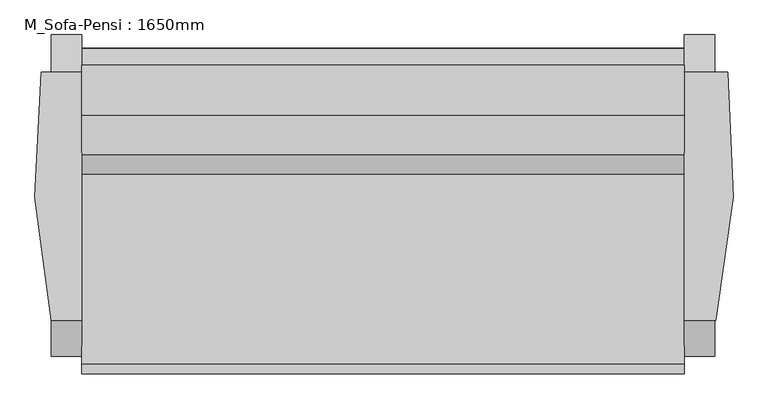
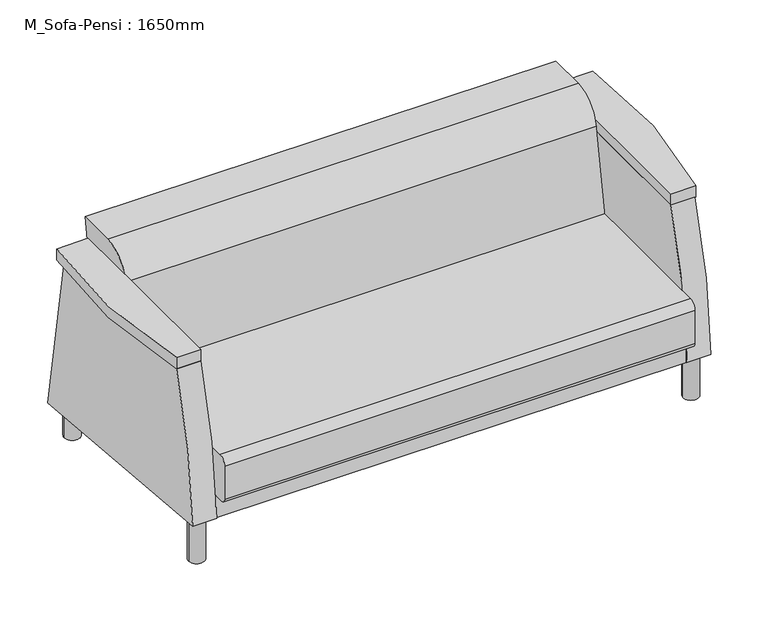
"""IFC4 building model written with IfcOpenShell, lengths in millimetres: furniture geometry, M_Sofa-Pensi : 1650mm."""

from ifc_helpers import new_model, si_unit, point, frame, frame_2d, origin, origin_with_axes, place, context, project, spatial, polyline, circle_curve, trimmed, segment, composite_curve, outline, extrude, source, transform, mapped, element, save
from ifc_brep_helpers import plane_surface, cylinder_surface, advanced_brep


def m_sofa_pensi_1650mm_31461fb8(model_context):
    return source(origin(), model_context, "Body", "SolidModel", [
        advanced_brep(
        [(1103.60625, 701.7619204, 79.3588346), (1103.60625, 608.6917937, 626.0203985), (1103.60625, -9.3943348, 626.0203985), (1103.60625, -97.7900405, 149.3105671), (1027.40625, -9.3943348, 626.0203985), (1027.40625, 608.6917937, 626.0203985), (1027.40625, 701.7619204, 79.3588346), (1027.40625, -83.3930704, 148.0509954), (1027.40625, 668.3047863, 148.0509954), (1027.40625, 668.3047863, 224.2509954), (1027.40625, -93.6952137, 224.2509954), (1027.40625, -93.6952137, 148.9523161), (1027.40625, -97.7900405, 149.3105671), (1027.40625, -93.6952137, 148.0509954), (-470.19375, -83.3930704, 148.0509954), (-470.19375, -93.6952137, 148.0509954), (-470.19375, -93.6952137, 148.9523161), (-470.19375, 668.3047863, 224.2509954), (-470.19375, -93.6952137, 224.2509954), (-470.19375, 668.3047863, 148.0509954), (-470.19375, 701.7619204, 79.3588346), (-470.19375, 608.6917937, 626.0203985), (-470.19375, -9.3943348, 626.0203985), (-470.19375, -97.7900405, 149.3105671), (-546.39375, -9.3943348, 626.0203985), (-546.39375, 608.6917937, 626.0203985), (-546.39375, 701.7619204, 79.3588346), (-546.39375, -97.7900405, 149.3105671)],
        [
            (0, 1),
            (1, 2),
            (2, 3, circle_curve(frame((1103.60625, 1499.9783711, 99.5888442), z_axis=(1.0, 0.0, 0.0), x_axis=(0.0, 1.0, 0.0)), 1598.5418814)),
            (3, 0),
            (4, 5),
            (5, 6),
            (6, 7),
            (7, 8),
            (8, 9),
            (9, 10),
            (10, 4, circle_curve(frame((1027.40625, 1499.9783711, 99.5888442), z_axis=(-1.0, 0.0, 0.0), x_axis=(0.0, 1.0, 0.0)), 1598.5418814)),
            (11, 12),
            (12, 10, circle_curve(frame((1027.40625, 1499.9783711, 99.5888442), z_axis=(-1.0, 0.0, 0.0), x_axis=(0.0, 1.0, 0.0)), 1598.5418814)),
            (10, 11),
            (0, 6),
            (5, 1),
            (4, 2),
            (12, 3),
            (11, 7),
            (11, 13),
            (13, 7),
            (14, 15),
            (15, 16),
            (16, 14),
            (9, 17),
            (17, 18),
            (18, 10),
            (18, 16),
            (15, 13),
            (14, 19),
            (19, 8),
            (19, 17),
            (20, 21),
            (21, 22),
            (22, 18, circle_curve(frame((-470.19375, 1499.9783711, 99.5888442), z_axis=(1.0, 0.0, 0.0), x_axis=(0.0, 1.0, 0.0)), 1598.5418814)),
            (14, 20),
            (18, 23, circle_curve(frame((-470.19375, 1499.9783711, 99.5888442), z_axis=(1.0, 0.0, 0.0), x_axis=(0.0, 1.0, 0.0)), 1598.5418814)),
            (23, 16),
            (24, 25),
            (25, 26),
            (26, 27),
            (27, 24, circle_curve(frame((-546.39375, 1499.9783711, 99.5888442), z_axis=(-1.0, 0.0, 0.0), x_axis=(0.0, 1.0, 0.0)), 1598.5418814)),
            (27, 23),
            (22, 24),
            (26, 20),
            (25, 21),
        ],
        [
            plane_surface(frame((1103.60625, 608.6917937, 626.0203985), z_axis=(1.0000000000000002, 0.0, 0.0), x_axis=(0.0, -0.16783676484789783, 0.985814800236531))),
            plane_surface(frame((1027.40625, 608.6917937, 626.0203985), z_axis=(-1.0000000000000002, 0.0, 0.0), x_axis=(0.0, 0.16783676484789783, -0.985814800236531))),
            plane_surface(frame((1103.60625, 701.7619204, 79.3588346), z_axis=(0.0, 0.985814800236531, 0.16783676484789783), x_axis=(-1.0, 0.0, 0.0))),
            plane_surface(frame((1103.60625, 608.6917937, 626.0203985), z_axis=(0.0, 0.0, 1.0), x_axis=(-1.0, 0.0, 0.0))),
            cylinder_surface(frame((1027.40625, 1499.9783711, 99.5888442), z_axis=(1.0, 0.0, 0.0), x_axis=(0.0, 1.0, 0.0)), 1598.5418814),
            plane_surface(frame((1103.60625, -97.7900405, 149.3105671), z_axis=(0.0, -0.08715574274767213, -0.9961946980917444), x_axis=(-1.0, 0.0, 0.0))),
            plane_surface(frame((1027.40625, -93.6952137, 224.2509954), z_axis=(1.0, 0.0, 0.0), x_axis=(0.0, -1.0, 0.0))),
            plane_surface(frame((-470.19375, -93.6952137, 224.2509954), z_axis=(-1.0, 0.0, 0.0), x_axis=(0.0, 1.0, 0.0))),
            plane_surface(frame((1027.40625, 668.3047863, 224.2509954), z_axis=(0.0, 0.0, 1.0), x_axis=(-1.0, 0.0, 0.0))),
            plane_surface(frame((1027.40625, -93.6952137, 224.2509954), z_axis=(0.0, -1.0, 0.0), x_axis=(-1.0, 0.0, 0.0))),
            plane_surface(frame((1027.40625, -93.6952137, 148.0509954), z_axis=(0.0, 0.0, -1.0), x_axis=(-1.0, 0.0, 0.0))),
            plane_surface(frame((1027.40625, 668.3047863, 148.0509954), z_axis=(0.0, 1.0, 0.0), x_axis=(-1.0, 0.0, 0.0))),
            plane_surface(frame((-470.19375, 3098.5202525, 99.5888442), z_axis=(1.0, 0.0, 0.0), x_axis=(0.0, 0.0, 1.0))),
            plane_surface(frame((-546.39375, 3098.5202525, 99.5888442), z_axis=(-1.0, 0.0, 0.0), x_axis=(0.0, 0.0, -1.0))),
            cylinder_surface(frame((-546.39375, 1499.9783711, 99.5888442), z_axis=(1.0, 0.0, 0.0), x_axis=(0.0, 1.0, 0.0)), 1598.5418814),
            plane_surface(frame((-470.19375, -97.7900405, 149.3105671), z_axis=(0.0, -0.08715574274766119, -0.9961946980917453), x_axis=(-1.0, 0.0, 0.0))),
            plane_surface(frame((-470.19375, 701.7619204, 79.3588346), z_axis=(0.0, 0.9858148002365317, 0.16783676484789398), x_axis=(-1.0, 0.0, 0.0))),
            plane_surface(frame((-470.19375, 608.6917937, 626.0203985), z_axis=(0.0, 0.0, 1.0), x_axis=(-1.0, 0.0, 0.0))),
        ],
        [
            (0, [[1, 2, 3, 4]]),
            (1, [[5, 6, 7, 8, 9, 10, 11]]),
            (1, [[12, 13, 14]]),
            (2, [[-1, 15, -6, 16]]),
            (3, [[-2, -16, -5, 17]]),
            (4, [[-3, -17, -11, -13, 18]]),
            (5, [[-4, -18, -12, 19, -7, -15]]),
            (6, [[20, 21, -19]]),
            (7, [[22, 23, 24]]),
            (8, [[25, 26, 27, -10]]),
            (9, [[-27, 28, -23, 29, -20, -14]]),
            (10, [[-29, -22, 30, 31, -8, -21]]),
            (11, [[-25, -9, -31, 32]]),
            (12, [[33, 34, 35, -26, -32, -30, 36]]),
            (12, [[37, 38, -28]]),
            (13, [[39, 40, 41, 42]]),
            (14, [[-42, 43, -37, -35, 44]]),
            (15, [[-41, 45, -36, -24, -38, -43]]),
            (16, [[-33, -45, -40, 46]]),
            (17, [[-34, -46, -39, -44]]),
        ],
    ),
        extrude(outline(composite_curve([segment(trimmed(circle_curve(frame_2d((-508.29375, -53.0901639)), 25.4), [point((-533.69375, -53.0901639))], [point((-482.89375, -53.0901639))], False, "CARTESIAN"), True, "CONTINUOUS"), segment(trimmed(circle_curve(frame_2d((-508.29375, -53.0901639)), 25.4), [point((-482.89375, -53.0901639))], [point((-533.69375, -53.0901639))], False, "CARTESIAN"), True, "CONTINUOUS")], self_intersect=False)), origin_with_axes(), (0.0, 0.0, 1.0), 148.43125),
        extrude(outline(composite_curve([segment(trimmed(circle_curve(frame_2d((-508.29375, 632.7098361)), 25.4), [point((-533.69375, 632.7098361))], [point((-482.89375, 632.7098361))], False, "CARTESIAN"), True, "CONTINUOUS"), segment(trimmed(circle_curve(frame_2d((-508.29375, 632.7098361)), 25.4), [point((-482.89375, 632.7098361))], [point((-533.69375, 632.7098361))], False, "CARTESIAN"), True, "CONTINUOUS")], self_intersect=False)), origin_with_axes(), (0.0, 0.0, 1.0), 148.43125),
        extrude(outline(composite_curve([segment(trimmed(circle_curve(frame_2d((1065.50625, 632.7098361)), 25.4), [point((1040.10625, 632.7098361))], [point((1090.90625, 632.7098361))], False, "CARTESIAN"), True, "CONTINUOUS"), segment(trimmed(circle_curve(frame_2d((1065.50625, 632.7098361)), 25.4), [point((1090.90625, 632.7098361))], [point((1040.10625, 632.7098361))], False, "CARTESIAN"), True, "CONTINUOUS")], self_intersect=False)), origin_with_axes(), (0.0, 0.0, 1.0), 148.43125),
        extrude(outline(composite_curve([segment(trimmed(circle_curve(frame_2d((1065.50625, -53.0901639)), 25.4), [point((1040.10625, -53.0901639))], [point((1090.90625, -53.0901639))], False, "CARTESIAN"), True, "CONTINUOUS"), segment(trimmed(circle_curve(frame_2d((1065.50625, -53.0901639)), 25.4), [point((1090.90625, -53.0901639))], [point((1040.10625, -53.0901639))], False, "CARTESIAN"), True, "CONTINUOUS")], self_intersect=False)), origin_with_axes(), (0.0, 0.0, 1.0), 148.43125),
        extrude(outline(composite_curve([segment(trimmed(circle_curve(frame_2d((-116.5901639, 351.2509954)), 25.4), [point((-141.9901639, 351.2509954))], [point((-116.5901639, 376.6509954))], False, "CARTESIAN"), True, "CONTINUOUS"), segment(polyline([(-116.5901639, 376.6509954), (355.3895541, 376.6509954), (402.1988177, 642.1195211)]), True, "CONTINUOUS"), segment(trimmed(circle_curve(frame_2d((502.2552854, 624.4768662)), 101.6), [point((402.1988177, 642.1195211))], [point((502.2552854, 726.0768662))], False, "CARTESIAN"), True, "CONTINUOUS"), segment(polyline([(502.2552854, 726.0768662), (626.3344485, 726.0768662), (609.5377828, 620.1719187), (667.6541767, 224.2509954), (-126.1151639, 224.2509954)]), True, "CONTINUOUS"), segment(trimmed(circle_curve(frame_2d((-126.1151639, 240.1259954)), 15.875), [point((-126.1151639, 224.2509954))], [point((-141.9901639, 240.1259954))], False, "CARTESIAN"), True, "CONTINUOUS"), segment(polyline([(-141.9901639, 240.1259954), (-141.9901639, 351.2509954)]), True, "CONTINUOUS")], self_intersect=False)), frame((-470.19375, 0.0, 0.0), z_axis=(1.0, 0.0, 0.0), x_axis=(0.0, 1.0, 0.0)), (0.0, 0.0, 1.0), 1497.6),
        extrude(outline(composite_curve([segment(polyline([(-470.19375, -9.3943348), (-546.39375, -9.3943348)]), True, "CONTINUOUS"), segment(trimmed(circle_curve(frame_2d((1137.7527561, 369.3799517)), 1726.2153441), [point((-546.39375, -9.3943348))], [point((-571.79375, 608.6917935))], False, "CARTESIAN"), True, "CONTINUOUS"), segment(polyline([(-571.79375, 608.6917935), (-470.19375, 608.6917935), (-470.19375, -9.3943348)]), True, "CONTINUOUS")], self_intersect=False)), frame((0.0, 0.0, 626.0203985), z_axis=(0.0, 0.0, 1.0), x_axis=(1.0, 0.0, 0.0)), (0.0, 0.0, 1.0), 38.1),
        extrude(outline(composite_curve([segment(polyline([(1027.40625, -9.3943348), (1027.40625, 608.9395268), (1136.0864453, 608.9395268)]), True, "CONTINUOUS"), segment(trimmed(circle_curve(frame_2d((-579.5771494, 383.2634494)), 1730.4425047), [point((1136.0864453, 608.9395268))], [point((1105.7273117, -9.3943348))], False, "CARTESIAN"), True, "CONTINUOUS"), segment(polyline([(1105.7273117, -9.3943348), (1027.40625, -9.3943348)]), True, "CONTINUOUS")], self_intersect=False)), frame((0.0, 0.0, 626.0203985), z_axis=(0.0, 0.0, 1.0), x_axis=(1.0, 0.0, 0.0)), (0.0, 0.0, 1.0), 38.1),
    ])


if __name__ == "__main__":
    model = new_model("IFC4")
    model_context = context("Model", 3, world=origin())
    ifc_project = project(units=[si_unit("LENGTHUNIT", "METRE", prefix="MILLI")], contexts=[model_context])
    site = spatial("IfcSite", under=ifc_project)
    building = spatial("IfcBuilding", under=site)
    placement = place(None, origin())
    m_sofa_pensi_1650mm_shape = m_sofa_pensi_1650mm_31461fb8(model_context)
    element("IfcFurniture", 1, ObjectType="M_Sofa-Pensi : 1650mm", at=placement, inside=building, context=model_context, shape_type="MappedRepresentation", body=[
        mapped(m_sofa_pensi_1650mm_shape, transform((0.0, 0.0, 0.0), x_axis=(1.0, 0.0, 0.0), y_axis=(0.0, 1.0, 0.0), z_axis=(0.0, 0.0, 1.0))),
    ])
    save(model, "model.ifc")

# Revit data of these elements
# Project information
#   Project Issue Date = "Issue Date"
#   Project Status = "Project  Status"
#   Client Name = "Owner"
#   Project Address = "## Street\nCity, State  Zip"
#   Project Name = "Project Name"
#   Project Number = "Project  Number"
# Type "M_Sofa-Pensi : 1650mm"
#   Length = 1.65 m
#   Sofa Material = Linen, Beige
#   Frame Material = Steel, Chrome Plated
# Element 1 (IfcFurniture, "M_Sofa-Pensi : 1650mm")
#   Materials on its faces: "Linen, Beige", "Steel, Chrome Plated"
# Materials
#   "Linen, Beige": class "Textile", colour RGB 249 239 230, transparency 0, Description = "Linen, beige", Cost = 0
#   "Steel, Chrome Plated": class "Metal", colour RGB 244 244 244, transparency 0, Description = "Chromiuim plated steel", Cost = 0
